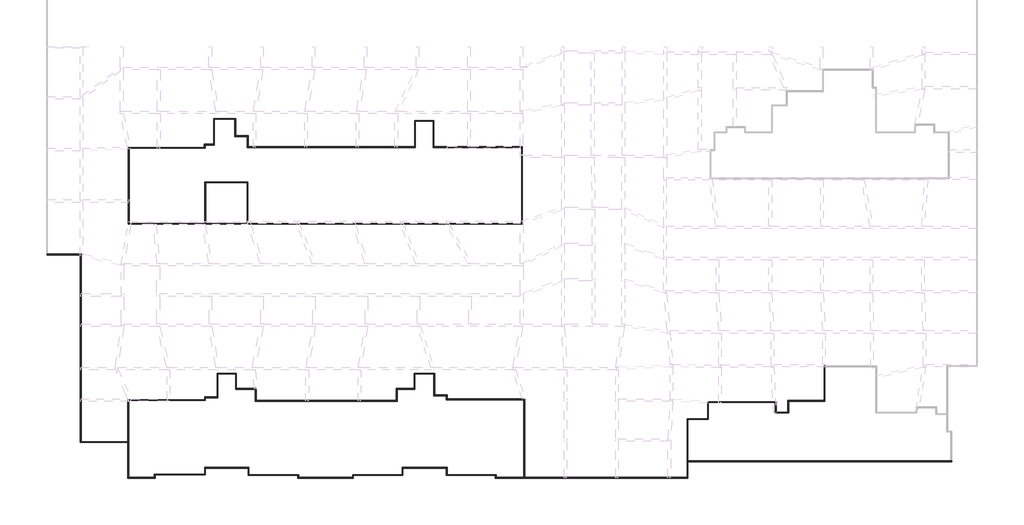
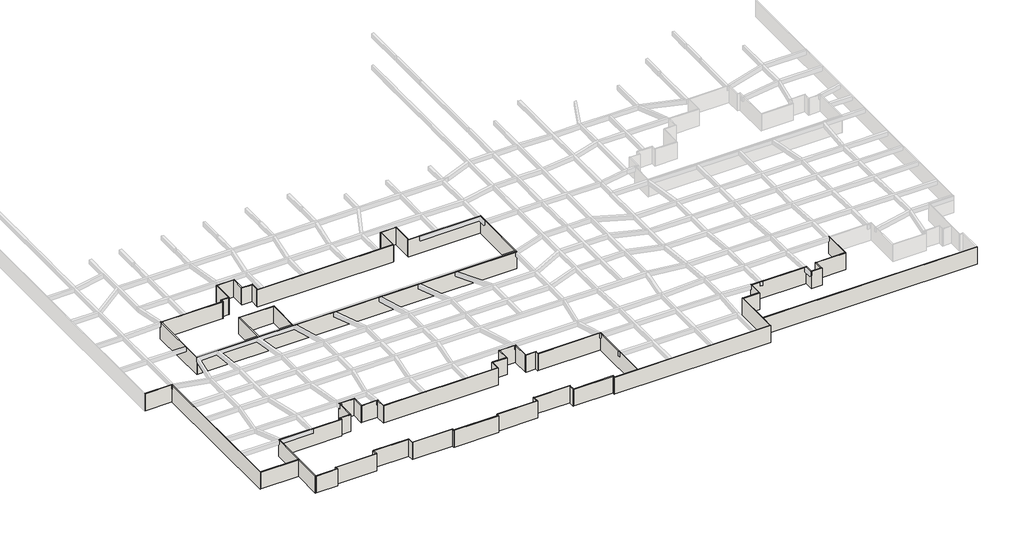
# One storey, part 1 of 45: 68 walls.
"""IFC4 building model written with IfcOpenShell, lengths in millimetres."""

from ifc_helpers import new_model, si_unit, origin, origin_with_axes, place, context, project, spatial, polyline, outline, extrude, faceted_brep, element, save

model = new_model("IFC4")

# Units and contexts
model_context = context("Model", 3, world=origin())
ifc_project = project(units=[si_unit("LENGTHUNIT", "METRE", prefix="MILLI")], contexts=[model_context])

# Site, building, storey
site = spatial("IfcSite", under=ifc_project)
building = spatial("IfcBuilding", under=site)
storey = spatial("IfcBuildingStorey", under=building, Name="户型图", Elevation=0.0)

# Walls
placement = place(None, origin())
element("IfcWall", 1, ObjectType="所有墙体", at=placement, inside=storey, context=model_context, shape_type="Brep", body=[
    faceted_brep([(-145580.5216564, -158288.0123265, 0.0), (-140600.5216564, -158288.0123265, 0.0), (-140480.5216564, -158288.0123265, 0.0), (-140480.5216564, -158288.0123265, 3300.0), (-140600.5216564, -158288.0123265, 3300.0), (-145580.5216564, -158288.0123265, 3300.0), (-145580.5216564, -158168.0123265, 0.0), (-145580.5216564, -158168.0123265, 3300.0), (-140480.5216564, -158168.0123265, 3300.0), (-140480.5216564, -158168.0123265, 0.0)], [[[0, 1, 2, 3, 4, 5]], [[6, 7, 8, 9]], [[2, 1, 0, 6, 9]], [[5, 4, 3, 8, 7]], [[0, 5, 7, 6]], [[3, 2, 9, 8]]]),
])
element("IfcWall", 2, ObjectType="所有墙体", at=placement, inside=storey, context=model_context, shape_type="Brep", body=[
    faceted_brep([(-140600.5216564, -158288.0123265, 0.0), (-140600.5216564, -186688.0123265, 0.0), (-140600.5216564, -186688.0123265, 3300.0), (-140600.5216564, -158288.0123265, 3300.0), (-140480.5216564, -158288.0123265, 0.0), (-140480.5216564, -158288.0123265, 3300.0), (-140480.5216564, -186568.0123265, 3300.0), (-140480.5216564, -186688.0123265, 3300.0), (-140480.5216564, -186688.0123265, 0.0), (-140480.5216564, -186568.0123265, 0.0)], [[[0, 1, 2, 3]], [[4, 5, 6, 7, 8, 9]], [[1, 0, 4, 9, 8]], [[3, 2, 7, 6, 5]], [[0, 3, 5, 4]], [[2, 1, 8, 7]]]),
])
element("IfcWall", 3, ObjectType="所有墙体", at=placement, inside=storey, context=model_context, shape_type="SweptSolid", body=[
    extrude(outline(polyline([(-133400.5216564, -186688.0123265), (-140480.5216564, -186688.0123265), (-140480.5216564, -186568.0123265), (-133400.5216564, -186568.0123265), (-133400.5216564, -186688.0123265)])), origin_with_axes(), (0.0, 0.0, 1.0), 3300.0),
])
element("IfcWall", 4, ObjectType="所有墙体", at=placement, inside=storey, context=model_context, shape_type="Brep", body=[
    faceted_brep([(-133400.5216564, -180210.4346237, 0.0), (-133400.5216564, -186568.0123265, 0.0), (-133400.5216564, -186688.0123265, 0.0), (-133400.5216564, -192088.0123265, 0.0), (-133400.5216564, -192088.0123265, 3300.0), (-133400.5216564, -186688.0123265, 3300.0), (-133400.5216564, -186568.0123265, 3300.0), (-133400.5216564, -180210.4346237, 3300.0), (-133280.5216564, -180210.4346237, 0.0), (-133280.5216564, -180210.4346237, 3300.0), (-133280.5216564, -180330.4346237, 3300.0), (-133280.5216564, -191968.0123265, 3300.0), (-133280.5216564, -192088.0123265, 3300.0), (-133280.5216564, -192088.0123265, 0.0), (-133280.5216564, -191968.0123265, 0.0), (-133280.5216564, -180330.4346237, 0.0)], [[[0, 1, 2, 3, 4, 5, 6, 7]], [[8, 9, 10, 11, 12, 13, 14, 15]], [[3, 2, 1, 0, 8, 15, 14, 13]], [[7, 6, 5, 4, 12, 11, 10, 9]], [[4, 3, 13, 12]], [[0, 7, 9, 8]]]),
])
element("IfcWall", 5, ObjectType="所有墙体", at=placement, inside=storey, context=model_context, shape_type="Brep", body=[
    faceted_brep([(-133280.5216564, -192088.0123265, 0.0), (-129280.5216564, -192088.0123265, 0.0), (-129280.5216564, -192088.0123265, 3300.0), (-133280.5216564, -192088.0123265, 3300.0), (-133280.5216564, -191968.0123265, 0.0), (-133280.5216564, -191968.0123265, 3300.0), (-129400.5216564, -191968.0123265, 3300.0), (-129280.5216564, -191968.0123265, 3300.0), (-129280.5216564, -191968.0123265, 0.0), (-129400.5216564, -191968.0123265, 0.0)], [[[0, 1, 2, 3]], [[4, 5, 6, 7, 8, 9]], [[1, 0, 4, 9, 8]], [[3, 2, 7, 6, 5]], [[0, 3, 5, 4]], [[2, 1, 8, 7]]]),
])
element("IfcWall", 6, ObjectType="所有墙体", at=placement, inside=storey, context=model_context, shape_type="Brep", body=[
    faceted_brep([(-129280.5216564, -191968.0123265, 0.0), (-129280.5216564, -191588.0123265, 0.0), (-129280.5216564, -191468.0123265, 0.0), (-129280.5216564, -191468.0123265, 3300.0), (-129280.5216564, -191588.0123265, 3300.0), (-129280.5216564, -191968.0123265, 3300.0), (-129400.5216564, -191968.0123265, 0.0), (-129400.5216564, -191968.0123265, 3300.0), (-129400.5216564, -191468.0123265, 3300.0), (-129400.5216564, -191468.0123265, 0.0)], [[[0, 1, 2, 3, 4, 5]], [[6, 7, 8, 9]], [[2, 1, 0, 6, 9]], [[5, 4, 3, 8, 7]], [[0, 5, 7, 6]], [[3, 2, 9, 8]]]),
])
element("IfcWall", 7, ObjectType="所有墙体", at=placement, inside=storey, context=model_context, shape_type="Brep", body=[
    faceted_brep([(-129280.5216564, -191588.0123265, 0.0), (-121680.5216564, -191588.0123265, 0.0), (-121680.5216564, -191588.0123265, 3300.0), (-129280.5216564, -191588.0123265, 3300.0), (-129280.5216564, -191468.0123265, 0.0), (-129280.5216564, -191468.0123265, 3300.0), (-121800.5216564, -191468.0123265, 3300.0), (-121680.5216564, -191468.0123265, 3300.0), (-121680.5216564, -191468.0123265, 0.0), (-121800.5216564, -191468.0123265, 0.0)], [[[0, 1, 2, 3]], [[4, 5, 6, 7, 8, 9]], [[1, 0, 4, 9, 8]], [[3, 2, 7, 6, 5]], [[0, 3, 5, 4]], [[2, 1, 8, 7]]]),
])
element("IfcWall", 8, ObjectType="所有墙体", at=placement, inside=storey, context=model_context, shape_type="Brep", body=[
    faceted_brep([(-121680.5216564, -191468.0123265, 0.0), (-121680.5216564, -190588.0123265, 0.0), (-121680.5216564, -190468.0123265, 0.0), (-121680.5216564, -190468.0123265, 3300.0), (-121680.5216564, -190588.0123265, 3300.0), (-121680.5216564, -191468.0123265, 3300.0), (-121800.5216564, -191468.0123265, 0.0), (-121800.5216564, -191468.0123265, 3300.0), (-121800.5216564, -190468.0123265, 3300.0), (-121800.5216564, -190468.0123265, 0.0)], [[[0, 1, 2, 3, 4, 5]], [[6, 7, 8, 9]], [[2, 1, 0, 6, 9]], [[5, 4, 3, 8, 7]], [[0, 5, 7, 6]], [[3, 2, 9, 8]]]),
])
element("IfcWall", 9, ObjectType="所有墙体", at=placement, inside=storey, context=model_context, shape_type="Brep", body=[
    faceted_brep([(-121680.5216564, -190588.0123265, 0.0), (-115200.5216564, -190588.0123265, 0.0), (-115080.5216564, -190588.0123265, 0.0), (-115080.5216564, -190588.0123265, 3300.0), (-115200.5216564, -190588.0123265, 3300.0), (-121680.5216564, -190588.0123265, 3300.0), (-121680.5216564, -190468.0123265, 0.0), (-121680.5216564, -190468.0123265, 3300.0), (-115080.5216564, -190468.0123265, 3300.0), (-115080.5216564, -190468.0123265, 0.0)], [[[0, 1, 2, 3, 4, 5]], [[6, 7, 8, 9]], [[2, 1, 0, 6, 9]], [[5, 4, 3, 8, 7]], [[0, 5, 7, 6]], [[3, 2, 9, 8]]]),
])
element("IfcWall", 10, ObjectType="所有墙体", at=placement, inside=storey, context=model_context, shape_type="Brep", body=[
    faceted_brep([(-115200.5216564, -190588.0123265, 0.0), (-115200.5216564, -191688.0123265, 0.0), (-115200.5216564, -191688.0123265, 3300.0), (-115200.5216564, -190588.0123265, 3300.0), (-115080.5216564, -190588.0123265, 0.0), (-115080.5216564, -190588.0123265, 3300.0), (-115080.5216564, -191568.0123265, 3300.0), (-115080.5216564, -191688.0123265, 3300.0), (-115080.5216564, -191688.0123265, 0.0), (-115080.5216564, -191568.0123265, 0.0)], [[[0, 1, 2, 3]], [[4, 5, 6, 7, 8, 9]], [[1, 0, 4, 9, 8]], [[3, 2, 7, 6, 5]], [[0, 3, 5, 4]], [[2, 1, 8, 7]]]),
])
element("IfcWall", 11, ObjectType="所有墙体", at=placement, inside=storey, context=model_context, shape_type="Brep", body=[
    faceted_brep([(-115080.5216564, -191688.0123265, 0.0), (-107700.5216564, -191688.0123265, 0.0), (-107580.5216564, -191688.0123265, 0.0), (-107580.5216564, -191688.0123265, 3300.0), (-107700.5216564, -191688.0123265, 3300.0), (-115080.5216564, -191688.0123265, 3300.0), (-115080.5216564, -191568.0123265, 0.0), (-115080.5216564, -191568.0123265, 3300.0), (-107580.5216564, -191568.0123265, 3300.0), (-107580.5216564, -191568.0123265, 0.0)], [[[0, 1, 2, 3, 4, 5]], [[6, 7, 8, 9]], [[2, 1, 0, 6, 9]], [[5, 4, 3, 8, 7]], [[0, 5, 7, 6]], [[3, 2, 9, 8]]]),
])
element("IfcWall", 12, ObjectType="所有墙体", at=placement, inside=storey, context=model_context, shape_type="Brep", body=[
    faceted_brep([(-107700.5216564, -191688.0123265, 0.0), (-107700.5216564, -192088.0123265, 0.0), (-107700.5216564, -192088.0123265, 3300.0), (-107700.5216564, -191688.0123265, 3300.0), (-107580.5216564, -191688.0123265, 0.0), (-107580.5216564, -191688.0123265, 3300.0), (-107580.5216564, -191968.0123265, 3300.0), (-107580.5216564, -192088.0123265, 3300.0), (-107580.5216564, -192088.0123265, 0.0), (-107580.5216564, -191968.0123265, 0.0)], [[[0, 1, 2, 3]], [[4, 5, 6, 7, 8, 9]], [[1, 0, 4, 9, 8]], [[3, 2, 7, 6, 5]], [[0, 3, 5, 4]], [[2, 1, 8, 7]]]),
])
element("IfcWall", 13, ObjectType="所有墙体", at=placement, inside=storey, context=model_context, shape_type="Brep", body=[
    faceted_brep([(-107580.5216564, -192088.0123265, 0.0), (-99280.5216564, -192088.0123265, 0.0), (-99280.5216564, -192088.0123265, 3300.0), (-107580.5216564, -192088.0123265, 3300.0), (-107580.5216564, -191968.0123265, 0.0), (-107580.5216564, -191968.0123265, 3300.0), (-99400.5216564, -191968.0123265, 3300.0), (-99280.5216564, -191968.0123265, 3300.0), (-99280.5216564, -191968.0123265, 0.0), (-99400.5216564, -191968.0123265, 0.0)], [[[0, 1, 2, 3]], [[4, 5, 6, 7, 8, 9]], [[1, 0, 4, 9, 8]], [[3, 2, 7, 6, 5]], [[0, 3, 5, 4]], [[2, 1, 8, 7]]]),
])
element("IfcWall", 14, ObjectType="所有墙体", at=placement, inside=storey, context=model_context, shape_type="Brep", body=[
    faceted_brep([(-99280.5216564, -191968.0123265, 0.0), (-99280.5216564, -191688.0123265, 0.0), (-99280.5216564, -191568.0123265, 0.0), (-99280.5216564, -191568.0123265, 3300.0), (-99280.5216564, -191688.0123265, 3300.0), (-99280.5216564, -191968.0123265, 3300.0), (-99400.5216564, -191968.0123265, 0.0), (-99400.5216564, -191968.0123265, 3300.0), (-99400.5216564, -191568.0123265, 3300.0), (-99400.5216564, -191568.0123265, 0.0)], [[[0, 1, 2, 3, 4, 5]], [[6, 7, 8, 9]], [[2, 1, 0, 6, 9]], [[5, 4, 3, 8, 7]], [[0, 5, 7, 6]], [[3, 2, 9, 8]]]),
])
element("IfcWall", 15, ObjectType="所有墙体", at=placement, inside=storey, context=model_context, shape_type="Brep", body=[
    faceted_brep([(-99280.5216564, -191688.0123265, 0.0), (-91780.5216564, -191688.0123265, 0.0), (-91780.5216564, -191688.0123265, 3300.0), (-99280.5216564, -191688.0123265, 3300.0), (-99280.5216564, -191568.0123265, 0.0), (-99280.5216564, -191568.0123265, 3300.0), (-91900.5216564, -191568.0123265, 3300.0), (-91780.5216564, -191568.0123265, 3300.0), (-91780.5216564, -191568.0123265, 0.0), (-91900.5216564, -191568.0123265, 0.0)], [[[0, 1, 2, 3]], [[4, 5, 6, 7, 8, 9]], [[1, 0, 4, 9, 8]], [[3, 2, 7, 6, 5]], [[0, 3, 5, 4]], [[2, 1, 8, 7]]]),
])
element("IfcWall", 16, ObjectType="所有墙体", at=placement, inside=storey, context=model_context, shape_type="Brep", body=[
    faceted_brep([(-91780.5216564, -191568.0123265, 0.0), (-91780.5216564, -190588.0123265, 0.0), (-91780.5216564, -190468.0123265, 0.0), (-91780.5216564, -190468.0123265, 3300.0), (-91780.5216564, -190588.0123265, 3300.0), (-91780.5216564, -191568.0123265, 3300.0), (-91900.5216564, -191568.0123265, 0.0), (-91900.5216564, -191568.0123265, 3300.0), (-91900.5216564, -190468.0123265, 3300.0), (-91900.5216564, -190468.0123265, 0.0)], [[[0, 1, 2, 3, 4, 5]], [[6, 7, 8, 9]], [[2, 1, 0, 6, 9]], [[5, 4, 3, 8, 7]], [[0, 5, 7, 6]], [[3, 2, 9, 8]]]),
])
element("IfcWall", 17, ObjectType="所有墙体", at=placement, inside=storey, context=model_context, shape_type="Brep", body=[
    faceted_brep([(-91780.5216564, -190588.0123265, 0.0), (-85200.5216564, -190588.0123265, 0.0), (-85080.5216564, -190588.0123265, 0.0), (-85080.5216564, -190588.0123265, 3300.0), (-85200.5216564, -190588.0123265, 3300.0), (-91780.5216564, -190588.0123265, 3300.0), (-91780.5216564, -190468.0123265, 0.0), (-91780.5216564, -190468.0123265, 3300.0), (-85080.5216564, -190468.0123265, 3300.0), (-85080.5216564, -190468.0123265, 0.0)], [[[0, 1, 2, 3, 4, 5]], [[6, 7, 8, 9]], [[2, 1, 0, 6, 9]], [[5, 4, 3, 8, 7]], [[0, 5, 7, 6]], [[3, 2, 9, 8]]]),
])
element("IfcWall", 18, ObjectType="所有墙体", at=placement, inside=storey, context=model_context, shape_type="Brep", body=[
    faceted_brep([(-85200.5216564, -190588.0123265, 0.0), (-85200.5216564, -191688.0123265, 0.0), (-85200.5216564, -191688.0123265, 3300.0), (-85200.5216564, -190588.0123265, 3300.0), (-85080.5216564, -190588.0123265, 0.0), (-85080.5216564, -190588.0123265, 3300.0), (-85080.5216564, -191568.0123265, 3300.0), (-85080.5216564, -191688.0123265, 3300.0), (-85080.5216564, -191688.0123265, 0.0), (-85080.5216564, -191568.0123265, 0.0)], [[[0, 1, 2, 3]], [[4, 5, 6, 7, 8, 9]], [[1, 0, 4, 9, 8]], [[3, 2, 7, 6, 5]], [[0, 3, 5, 4]], [[2, 1, 8, 7]]]),
])
element("IfcWall", 19, ObjectType="所有墙体", at=placement, inside=storey, context=model_context, shape_type="Brep", body=[
    faceted_brep([(-85080.5216564, -191688.0123265, 0.0), (-77800.5216564, -191688.0123265, 0.0), (-77680.5216564, -191688.0123265, 0.0), (-77680.5216564, -191688.0123265, 3300.0), (-77800.5216564, -191688.0123265, 3300.0), (-85080.5216564, -191688.0123265, 3300.0), (-85080.5216564, -191568.0123265, 0.0), (-85080.5216564, -191568.0123265, 3300.0), (-77680.5216564, -191568.0123265, 3300.0), (-77680.5216564, -191568.0123265, 0.0)], [[[0, 1, 2, 3, 4, 5]], [[6, 7, 8, 9]], [[2, 1, 0, 6, 9]], [[5, 4, 3, 8, 7]], [[0, 5, 7, 6]], [[3, 2, 9, 8]]]),
])
element("IfcWall", 20, ObjectType="所有墙体", at=placement, inside=storey, context=model_context, shape_type="Brep", body=[
    faceted_brep([(-77800.5216564, -191688.0123265, 0.0), (-77800.5216564, -192088.0123265, 0.0), (-77800.5216564, -192088.0123265, 3300.0), (-77800.5216564, -191688.0123265, 3300.0), (-77680.5216564, -191688.0123265, 0.0), (-77680.5216564, -191688.0123265, 3300.0), (-77680.5216564, -191968.0123265, 3300.0), (-77680.5216564, -192088.0123265, 3300.0), (-77680.5216564, -192088.0123265, 0.0), (-77680.5216564, -191968.0123265, 0.0)], [[[0, 1, 2, 3]], [[4, 5, 6, 7, 8, 9]], [[1, 0, 4, 9, 8]], [[3, 2, 7, 6, 5]], [[0, 3, 5, 4]], [[2, 1, 8, 7]]]),
])
element("IfcWall", 21, ObjectType="所有墙体", at=placement, inside=storey, context=model_context, shape_type="Brep", body=[
    faceted_brep([(-77680.5216564, -192088.0123265, 0.0), (-48680.5216564, -192088.0123265, 0.0), (-48680.5216564, -192088.0123265, 3300.0), (-77680.5216564, -192088.0123265, 3300.0), (-77680.5216564, -191968.0123265, 0.0), (-77680.5216564, -191968.0123265, 3300.0), (-73500.5216564, -191968.0123265, 3300.0), (-73380.5216564, -191968.0123265, 3300.0), (-48800.5216564, -191968.0123265, 3300.0), (-48680.5216564, -191968.0123265, 3300.0), (-48680.5216564, -191968.0123265, 0.0), (-48800.5216564, -191968.0123265, 0.0), (-73380.5216564, -191968.0123265, 0.0), (-73500.5216564, -191968.0123265, 0.0)], [[[0, 1, 2, 3]], [[4, 5, 6, 7, 8, 9, 10, 11, 12, 13]], [[1, 0, 4, 13, 12, 11, 10]], [[3, 2, 9, 8, 7, 6, 5]], [[0, 3, 5, 4]], [[2, 1, 10, 9]]]),
])
element("IfcWall", 22, ObjectType="所有墙体", at=placement, inside=storey, context=model_context, shape_type="Brep", body=[
    faceted_brep([(-48680.5216564, -191968.0123265, 0.0), (-48680.5216564, -189588.0123265, 0.0), (-48680.5216564, -189468.0123265, 0.0), (-48680.5216564, -183188.0123265, 0.0), (-48680.5216564, -183068.0123265, 0.0), (-48680.5216564, -183068.0123265, 3300.0), (-48680.5216564, -183188.0123265, 3300.0), (-48680.5216564, -189468.0123265, 3300.0), (-48680.5216564, -189588.0123265, 3300.0), (-48680.5216564, -191968.0123265, 3300.0), (-48800.5216564, -191968.0123265, 0.0), (-48800.5216564, -191968.0123265, 3300.0), (-48800.5216564, -183068.0123265, 3300.0), (-48800.5216564, -183068.0123265, 0.0)], [[[0, 1, 2, 3, 4, 5, 6, 7, 8, 9]], [[10, 11, 12, 13]], [[4, 3, 2, 1, 0, 10, 13]], [[9, 8, 7, 6, 5, 12, 11]], [[0, 9, 11, 10]], [[5, 4, 13, 12]]]),
])
element("IfcWall", 23, ObjectType="所有墙体", at=placement, inside=storey, context=model_context, shape_type="Brep", body=[
    faceted_brep([(-48680.5216564, -189588.0123265, 0.0), (-8780.5216564, -189588.0123265, 0.0), (-8780.5216564, -189588.0123265, 3300.0), (-48680.5216564, -189588.0123265, 3300.0), (-48680.5216564, -189468.0123265, 0.0), (-48680.5216564, -189468.0123265, 3300.0), (-8900.5216564, -189468.0123265, 3300.0), (-8780.5216564, -189468.0123265, 3300.0), (-8780.5216564, -189468.0123265, 0.0), (-8900.5216564, -189468.0123265, 0.0)], [[[0, 1, 2, 3]], [[4, 5, 6, 7, 8, 9]], [[1, 0, 4, 9, 8]], [[3, 2, 7, 6, 5]], [[0, 3, 5, 4]], [[2, 1, 8, 7]]]),
])
element("IfcWall", 24, ObjectType="所有墙体", at=placement, inside=storey, context=model_context, shape_type="Brep", body=[
    faceted_brep([(-133280.5216564, -180330.4346237, 0.0), (-121680.5216564, -180330.4346237, 0.0), (-121680.5216564, -180330.4346237, 3300.0), (-133280.5216564, -180330.4346237, 3300.0), (-133280.5216564, -180210.4346237, 0.0), (-133280.5216564, -180210.4346237, 3300.0), (-121800.5216564, -180210.4346237, 3300.0), (-121680.5216564, -180210.4346237, 3300.0), (-121680.5216564, -180210.4346237, 0.0), (-121800.5216564, -180210.4346237, 0.0)], [[[0, 1, 2, 3]], [[4, 5, 6, 7, 8, 9]], [[1, 0, 4, 9, 8]], [[3, 2, 7, 6, 5]], [[0, 3, 5, 4]], [[2, 1, 8, 7]]]),
])
element("IfcWall", 25, ObjectType="所有墙体", at=placement, inside=storey, context=model_context, shape_type="Brep", body=[
    faceted_brep([(-121680.5216564, -180210.4346237, 0.0), (-121680.5216564, -179930.4346237, 0.0), (-121680.5216564, -179810.4346237, 0.0), (-121680.5216564, -179810.4346237, 3300.0), (-121680.5216564, -179930.4346237, 3300.0), (-121680.5216564, -180210.4346237, 3300.0), (-121800.5216564, -180210.4346237, 0.0), (-121800.5216564, -180210.4346237, 3300.0), (-121800.5216564, -179810.4346237, 3300.0), (-121800.5216564, -179810.4346237, 0.0)], [[[0, 1, 2, 3, 4, 5]], [[6, 7, 8, 9]], [[2, 1, 0, 6, 9]], [[5, 4, 3, 8, 7]], [[0, 5, 7, 6]], [[3, 2, 9, 8]]]),
])
element("IfcWall", 26, ObjectType="所有墙体", at=placement, inside=storey, context=model_context, shape_type="Brep", body=[
    faceted_brep([(-121680.5216564, -179930.4346237, 0.0), (-119780.5216564, -179930.4346237, 0.0), (-119780.5216564, -179930.4346237, 3300.0), (-121680.5216564, -179930.4346237, 3300.0), (-121680.5216564, -179810.4346237, 0.0), (-121680.5216564, -179810.4346237, 3300.0), (-119900.5216564, -179810.4346237, 3300.0), (-119780.5216564, -179810.4346237, 3300.0), (-119780.5216564, -179810.4346237, 0.0), (-119900.5216564, -179810.4346237, 0.0)], [[[0, 1, 2, 3]], [[4, 5, 6, 7, 8, 9]], [[1, 0, 4, 9, 8]], [[3, 2, 7, 6, 5]], [[0, 3, 5, 4]], [[2, 1, 8, 7]]]),
])
element("IfcWall", 27, ObjectType="所有墙体", at=placement, inside=storey, context=model_context, shape_type="Brep", body=[
    faceted_brep([(-119780.5216564, -179810.4346237, 0.0), (-119780.5216564, -176330.4346237, 0.0), (-119780.5216564, -176210.4346237, 0.0), (-119780.5216564, -176210.4346237, 3300.0), (-119780.5216564, -176330.4346237, 3300.0), (-119780.5216564, -179810.4346237, 3300.0), (-119900.5216564, -179810.4346237, 0.0), (-119900.5216564, -179810.4346237, 3300.0), (-119900.5216564, -176210.4346237, 3300.0), (-119900.5216564, -176210.4346237, 0.0)], [[[0, 1, 2, 3, 4, 5]], [[6, 7, 8, 9]], [[2, 1, 0, 6, 9]], [[5, 4, 3, 8, 7]], [[0, 5, 7, 6]], [[3, 2, 9, 8]]]),
])
element("IfcWall", 28, ObjectType="所有墙体", at=placement, inside=storey, context=model_context, shape_type="Brep", body=[
    faceted_brep([(-119780.5216564, -176330.4346237, 0.0), (-117100.5216564, -176330.4346237, 0.0), (-116980.5216564, -176330.4346237, 0.0), (-116980.5216564, -176330.4346237, 3300.0), (-117100.5216564, -176330.4346237, 3300.0), (-119780.5216564, -176330.4346237, 3300.0), (-119780.5216564, -176210.4346237, 0.0), (-119780.5216564, -176210.4346237, 3300.0), (-116980.5216564, -176210.4346237, 3300.0), (-116980.5216564, -176210.4346237, 0.0)], [[[0, 1, 2, 3, 4, 5]], [[6, 7, 8, 9]], [[2, 1, 0, 6, 9]], [[5, 4, 3, 8, 7]], [[0, 5, 7, 6]], [[3, 2, 9, 8]]]),
])
element("IfcWall", 29, ObjectType="所有墙体", at=placement, inside=storey, context=model_context, shape_type="Brep", body=[
    faceted_brep([(-117100.5216564, -176330.4346237, 0.0), (-117100.5216564, -178630.4346237, 0.0), (-117100.5216564, -178630.4346237, 3300.0), (-117100.5216564, -176330.4346237, 3300.0), (-116980.5216564, -176330.4346237, 0.0), (-116980.5216564, -176330.4346237, 3300.0), (-116980.5216564, -178510.4346237, 3300.0), (-116980.5216564, -178630.4346237, 3300.0), (-116980.5216564, -178630.4346237, 0.0), (-116980.5216564, -178510.4346237, 0.0)], [[[0, 1, 2, 3]], [[4, 5, 6, 7, 8, 9]], [[1, 0, 4, 9, 8]], [[3, 2, 7, 6, 5]], [[0, 3, 5, 4]], [[2, 1, 8, 7]]]),
])
element("IfcWall", 30, ObjectType="所有墙体", at=placement, inside=storey, context=model_context, shape_type="Brep", body=[
    faceted_brep([(-116980.5216564, -178630.4346237, 0.0), (-114100.5216564, -178630.4346237, 0.0), (-113980.5216564, -178630.4346237, 0.0), (-113980.5216564, -178630.4346237, 3300.0), (-114100.5216564, -178630.4346237, 3300.0), (-116980.5216564, -178630.4346237, 3300.0), (-116980.5216564, -178510.4346237, 0.0), (-116980.5216564, -178510.4346237, 3300.0), (-113980.5216564, -178510.4346237, 3300.0), (-113980.5216564, -178510.4346237, 0.0)], [[[0, 1, 2, 3, 4, 5]], [[6, 7, 8, 9]], [[2, 1, 0, 6, 9]], [[5, 4, 3, 8, 7]], [[0, 5, 7, 6]], [[3, 2, 9, 8]]]),
])
element("IfcWall", 31, ObjectType="所有墙体", at=placement, inside=storey, context=model_context, shape_type="Brep", body=[
    faceted_brep([(-114100.5216564, -178630.4346237, 0.0), (-114100.5216564, -180430.4346237, 0.0), (-114100.5216564, -180430.4346237, 3300.0), (-114100.5216564, -178630.4346237, 3300.0), (-113980.5216564, -178630.4346237, 0.0), (-113980.5216564, -178630.4346237, 3300.0), (-113980.5216564, -180310.4346237, 3300.0), (-113980.5216564, -180430.4346237, 3300.0), (-113980.5216564, -180430.4346237, 0.0), (-113980.5216564, -180310.4346237, 0.0)], [[[0, 1, 2, 3]], [[4, 5, 6, 7, 8, 9]], [[1, 0, 4, 9, 8]], [[3, 2, 7, 6, 5]], [[0, 3, 5, 4]], [[2, 1, 8, 7]]]),
])
element("IfcWall", 32, ObjectType="所有墙体", at=placement, inside=storey, context=model_context, shape_type="Brep", body=[
    faceted_brep([(-113980.5216564, -180430.4346237, 0.0), (-92680.5216564, -180430.4346237, 0.0), (-92680.5216564, -180430.4346237, 3300.0), (-113980.5216564, -180430.4346237, 3300.0), (-113980.5216564, -180310.4346237, 0.0), (-113980.5216564, -180310.4346237, 3300.0), (-92800.5216564, -180310.4346237, 3300.0), (-92680.5216564, -180310.4346237, 3300.0), (-92680.5216564, -180310.4346237, 0.0), (-92800.5216564, -180310.4346237, 0.0)], [[[0, 1, 2, 3]], [[4, 5, 6, 7, 8, 9]], [[1, 0, 4, 9, 8]], [[3, 2, 7, 6, 5]], [[0, 3, 5, 4]], [[2, 1, 8, 7]]]),
])
element("IfcWall", 33, ObjectType="所有墙体", at=placement, inside=storey, context=model_context, shape_type="Brep", body=[
    faceted_brep([(-92680.5216564, -180310.4346237, 0.0), (-92680.5216564, -178630.4346237, 0.0), (-92680.5216564, -178510.4346237, 0.0), (-92680.5216564, -178510.4346237, 3300.0), (-92680.5216564, -178630.4346237, 3300.0), (-92680.5216564, -180310.4346237, 3300.0), (-92800.5216564, -180310.4346237, 0.0), (-92800.5216564, -180310.4346237, 3300.0), (-92800.5216564, -178510.4346237, 3300.0), (-92800.5216564, -178510.4346237, 0.0)], [[[0, 1, 2, 3, 4, 5]], [[6, 7, 8, 9]], [[2, 1, 0, 6, 9]], [[5, 4, 3, 8, 7]], [[0, 5, 7, 6]], [[3, 2, 9, 8]]]),
])
element("IfcWall", 34, ObjectType="所有墙体", at=placement, inside=storey, context=model_context, shape_type="Brep", body=[
    faceted_brep([(-92680.5216564, -178630.4346237, 0.0), (-89980.5216564, -178630.4346237, 0.0), (-89980.5216564, -178630.4346237, 3300.0), (-92680.5216564, -178630.4346237, 3300.0), (-92680.5216564, -178510.4346237, 0.0), (-92680.5216564, -178510.4346237, 3300.0), (-90100.5216564, -178510.4346237, 3300.0), (-89980.5216564, -178510.4346237, 3300.0), (-89980.5216564, -178510.4346237, 0.0), (-90100.5216564, -178510.4346237, 0.0)], [[[0, 1, 2, 3]], [[4, 5, 6, 7, 8, 9]], [[1, 0, 4, 9, 8]], [[3, 2, 7, 6, 5]], [[0, 3, 5, 4]], [[2, 1, 8, 7]]]),
])
element("IfcWall", 35, ObjectType="所有墙体", at=placement, inside=storey, context=model_context, shape_type="Brep", body=[
    faceted_brep([(-89980.5216564, -178510.4346237, 0.0), (-89980.5216564, -176330.4346237, 0.0), (-89980.5216564, -176210.4346237, 0.0), (-89980.5216564, -176210.4346237, 3300.0), (-89980.5216564, -176330.4346237, 3300.0), (-89980.5216564, -178510.4346237, 3300.0), (-90100.5216564, -178510.4346237, 0.0), (-90100.5216564, -178510.4346237, 3300.0), (-90100.5216564, -176210.4346237, 3300.0), (-90100.5216564, -176210.4346237, 0.0)], [[[0, 1, 2, 3, 4, 5]], [[6, 7, 8, 9]], [[2, 1, 0, 6, 9]], [[5, 4, 3, 8, 7]], [[0, 5, 7, 6]], [[3, 2, 9, 8]]]),
])
element("IfcWall", 36, ObjectType="所有墙体", at=placement, inside=storey, context=model_context, shape_type="Brep", body=[
    faceted_brep([(-89980.5216564, -176330.4346237, 0.0), (-87098.9727528, -176330.4346237, 0.0), (-86978.9727528, -176330.4346237, 0.0), (-86978.9727528, -176330.4346237, 3300.0), (-87098.9727528, -176330.4346237, 3300.0), (-89980.5216564, -176330.4346237, 3300.0), (-89980.5216564, -176210.4346237, 0.0), (-89980.5216564, -176210.4346237, 3300.0), (-86978.9727528, -176210.4346237, 3300.0), (-86978.9727528, -176210.4346237, 0.0)], [[[0, 1, 2, 3, 4, 5]], [[6, 7, 8, 9]], [[2, 1, 0, 6, 9]], [[5, 4, 3, 8, 7]], [[0, 5, 7, 6]], [[3, 2, 9, 8]]]),
])
element("IfcWall", 37, ObjectType="所有墙体", at=placement, inside=storey, context=model_context, shape_type="SweptSolid", body=[
    extrude(outline(polyline([(-87098.9727528, -179475.6864738), (-87098.9727528, -176330.4346237), (-86978.9727528, -176330.4346237), (-86978.9727528, -179475.6864738), (-87098.9727528, -179475.6864738)])), origin_with_axes(), (0.0, 0.0, 1.0), 3300.0),
])
element("IfcWall", 38, ObjectType="所有墙体", at=placement, inside=storey, context=model_context, shape_type="Brep", body=[
    faceted_brep([(-87098.9727528, -179595.6864738, 0.0), (-85200.5216564, -179595.6864738, 0.0), (-85080.5216564, -179595.6864738, 0.0), (-85080.5216564, -179595.6864738, 3300.0), (-85200.5216564, -179595.6864738, 3300.0), (-87098.9727528, -179595.6864738, 3300.0), (-87098.9727528, -179475.6864738, 0.0), (-87098.9727528, -179475.6864738, 3300.0), (-86978.9727528, -179475.6864738, 3300.0), (-85080.5216564, -179475.6864738, 3300.0), (-85080.5216564, -179475.6864738, 0.0), (-86978.9727528, -179475.6864738, 0.0)], [[[0, 1, 2, 3, 4, 5]], [[6, 7, 8, 9, 10, 11]], [[2, 1, 0, 6, 11, 10]], [[5, 4, 3, 9, 8, 7]], [[3, 2, 10, 9]], [[0, 5, 7, 6]]]),
])
element("IfcWall", 39, ObjectType="所有墙体", at=placement, inside=storey, context=model_context, shape_type="Brep", body=[
    faceted_brep([(-85200.5216564, -179595.6864738, 0.0), (-85200.5216564, -180195.6864738, 0.0), (-85200.5216564, -180195.6864738, 3300.0), (-85200.5216564, -179595.6864738, 3300.0), (-85080.5216564, -179595.6864738, 0.0), (-85080.5216564, -179595.6864738, 3300.0), (-85080.5216564, -180075.6864738, 3300.0), (-85080.5216564, -180195.6864738, 3300.0), (-85080.5216564, -180195.6864738, 0.0), (-85080.5216564, -180075.6864738, 0.0)], [[[0, 1, 2, 3]], [[4, 5, 6, 7, 8, 9]], [[1, 0, 4, 9, 8]], [[3, 2, 7, 6, 5]], [[0, 3, 5, 4]], [[2, 1, 8, 7]]]),
])
element("IfcWall", 40, ObjectType="所有墙体", at=placement, inside=storey, context=model_context, shape_type="Brep", body=[
    faceted_brep([(-85080.5216564, -180195.6864738, 0.0), (-73500.5216564, -180195.6864738, 0.0), (-73380.5216564, -180195.6864738, 0.0), (-73380.5216564, -180195.6864738, 3300.0), (-73500.5216564, -180195.6864738, 3300.0), (-85080.5216564, -180195.6864738, 3300.0), (-85080.5216564, -180075.6864738, 0.0), (-85080.5216564, -180075.6864738, 3300.0), (-73380.5216564, -180075.6864738, 3300.0), (-73380.5216564, -180075.6864738, 0.0)], [[[0, 1, 2, 3, 4, 5]], [[6, 7, 8, 9]], [[2, 1, 0, 6, 9]], [[5, 4, 3, 8, 7]], [[0, 5, 7, 6]], [[3, 2, 9, 8]]]),
])
element("IfcWall", 41, ObjectType="所有墙体", at=placement, inside=storey, context=model_context, shape_type="SweptSolid", body=[
    extrude(outline(polyline([(-73500.5216564, -191968.0123265), (-73500.5216564, -180195.6864738), (-73380.5216564, -180195.6864738), (-73380.5216564, -191968.0123265), (-73500.5216564, -191968.0123265)])), origin_with_axes(), (0.0, 0.0, 1.0), 3300.0),
])
element("IfcWall", 42, ObjectType="所有墙体", at=placement, inside=storey, context=model_context, shape_type="Brep", body=[
    faceted_brep([(-48680.5216564, -183188.0123265, 0.0), (-45580.5216564, -183188.0123265, 0.0), (-45580.5216564, -183188.0123265, 3300.0), (-48680.5216564, -183188.0123265, 3300.0), (-48680.5216564, -183068.0123265, 0.0), (-48680.5216564, -183068.0123265, 3300.0), (-45700.5216564, -183068.0123265, 3300.0), (-45580.5216564, -183068.0123265, 3300.0), (-45580.5216564, -183068.0123265, 0.0), (-45700.5216564, -183068.0123265, 0.0)], [[[0, 1, 2, 3]], [[4, 5, 6, 7, 8, 9]], [[1, 0, 4, 9, 8]], [[3, 2, 7, 6, 5]], [[0, 3, 5, 4]], [[2, 1, 8, 7]]]),
])
element("IfcWall", 43, ObjectType="所有墙体", at=placement, inside=storey, context=model_context, shape_type="Brep", body=[
    faceted_brep([(-45580.5216564, -183068.0123265, 0.0), (-45580.5216564, -180621.8863426, 0.0), (-45580.5216564, -180501.8863426, 0.0), (-45580.5216564, -180501.8863426, 3300.0), (-45580.5216564, -180621.8863426, 3300.0), (-45580.5216564, -183068.0123265, 3300.0), (-45700.5216564, -183068.0123265, 0.0), (-45700.5216564, -183068.0123265, 3300.0), (-45700.5216564, -180501.8863426, 3300.0), (-45700.5216564, -180501.8863426, 0.0)], [[[0, 1, 2, 3, 4, 5]], [[6, 7, 8, 9]], [[2, 1, 0, 6, 9]], [[5, 4, 3, 8, 7]], [[0, 5, 7, 6]], [[3, 2, 9, 8]]]),
])
element("IfcWall", 44, ObjectType="所有墙体", at=placement, inside=storey, context=model_context, shape_type="Brep", body=[
    faceted_brep([(-45580.5216564, -180621.8863426, 0.0), (-35471.0528269, -180621.8863426, 0.0), (-35351.0528269, -180621.8863426, 0.0), (-35351.0528269, -180621.8863426, 3300.0), (-35471.0528269, -180621.8863426, 3300.0), (-45580.5216564, -180621.8863426, 3300.0), (-45580.5216564, -180501.8863426, 0.0), (-45580.5216564, -180501.8863426, 3300.0), (-35351.0528269, -180501.8863426, 3300.0), (-35351.0528269, -180501.8863426, 0.0)], [[[0, 1, 2, 3, 4, 5]], [[6, 7, 8, 9]], [[2, 1, 0, 6, 9]], [[5, 4, 3, 8, 7]], [[0, 5, 7, 6]], [[3, 2, 9, 8]]]),
])
element("IfcWall", 45, ObjectType="所有墙体", at=placement, inside=storey, context=model_context, shape_type="Brep", body=[
    faceted_brep([(-35471.0528269, -180621.8863426, 0.0), (-35471.0528269, -182221.8863426, 0.0), (-35471.0528269, -182221.8863426, 3300.0), (-35471.0528269, -180621.8863426, 3300.0), (-35351.0528269, -180621.8863426, 0.0), (-35351.0528269, -180621.8863426, 3300.0), (-35351.0528269, -182101.8863426, 3300.0), (-35351.0528269, -182221.8863426, 3300.0), (-35351.0528269, -182221.8863426, 0.0), (-35351.0528269, -182101.8863426, 0.0)], [[[0, 1, 2, 3]], [[4, 5, 6, 7, 8, 9]], [[1, 0, 4, 9, 8]], [[3, 2, 7, 6, 5]], [[0, 3, 5, 4]], [[2, 1, 8, 7]]]),
])
element("IfcWall", 46, ObjectType="所有墙体", at=placement, inside=storey, context=model_context, shape_type="Brep", body=[
    faceted_brep([(-35351.0528269, -182221.8863426, 0.0), (-33451.0528269, -182221.8863426, 0.0), (-33451.0528269, -182221.8863426, 3300.0), (-35351.0528269, -182221.8863426, 3300.0), (-35351.0528269, -182101.8863426, 0.0), (-35351.0528269, -182101.8863426, 3300.0), (-33571.0528269, -182101.8863426, 3300.0), (-33451.0528269, -182101.8863426, 3300.0), (-33451.0528269, -182101.8863426, 0.0), (-33571.0528269, -182101.8863426, 0.0)], [[[0, 1, 2, 3]], [[4, 5, 6, 7, 8, 9]], [[1, 0, 4, 9, 8]], [[3, 2, 7, 6, 5]], [[0, 3, 5, 4]], [[2, 1, 8, 7]]]),
])
element("IfcWall", 47, ObjectType="所有墙体", at=placement, inside=storey, context=model_context, shape_type="Brep", body=[
    faceted_brep([(-33451.0528269, -182101.8863426, 0.0), (-33451.0528269, -180421.8863426, 0.0), (-33451.0528269, -180301.8863426, 0.0), (-33451.0528269, -180301.8863426, 3300.0), (-33451.0528269, -180421.8863426, 3300.0), (-33451.0528269, -182101.8863426, 3300.0), (-33571.0528269, -182101.8863426, 0.0), (-33571.0528269, -182101.8863426, 3300.0), (-33571.0528269, -180301.8863426, 3300.0), (-33571.0528269, -180301.8863426, 0.0)], [[[0, 1, 2, 3, 4, 5]], [[6, 7, 8, 9]], [[2, 1, 0, 6, 9]], [[5, 4, 3, 8, 7]], [[0, 5, 7, 6]], [[3, 2, 9, 8]]]),
])
element("IfcWall", 48, ObjectType="所有墙体", at=placement, inside=storey, context=model_context, shape_type="Brep", body=[
    faceted_brep([(-33451.0528269, -180421.8863426, 0.0), (-27951.0528269, -180421.8863426, 0.0), (-27951.0528269, -180421.8863426, 3300.0), (-33451.0528269, -180421.8863426, 3300.0), (-33451.0528269, -180301.8863426, 0.0), (-33451.0528269, -180301.8863426, 3300.0), (-28071.0528269, -180301.8863426, 3300.0), (-27951.0528269, -180301.8863426, 3300.0), (-27951.0528269, -180301.8863426, 0.0), (-28071.0528269, -180301.8863426, 0.0)], [[[0, 1, 2, 3]], [[4, 5, 6, 7, 8, 9]], [[1, 0, 4, 9, 8]], [[3, 2, 7, 6, 5]], [[0, 3, 5, 4]], [[2, 1, 8, 7]]]),
])
element("IfcWall", 49, ObjectType="所有墙体", at=placement, inside=storey, context=model_context, shape_type="Brep", body=[
    faceted_brep([(-27951.0528269, -180301.8863426, 0.0), (-27951.0528269, -175221.8863426, 0.0), (-27951.0528269, -175101.8863426, 0.0), (-27951.0528269, -175101.8863426, 3300.0), (-27951.0528269, -175221.8863426, 3300.0), (-27951.0528269, -180301.8863426, 3300.0), (-28071.0528269, -180301.8863426, 0.0), (-28071.0528269, -180301.8863426, 3300.0), (-28071.0528269, -175101.8863426, 3300.0), (-28071.0528269, -175101.8863426, 0.0)], [[[0, 1, 2, 3, 4, 5]], [[6, 7, 8, 9]], [[2, 1, 0, 6, 9]], [[5, 4, 3, 8, 7]], [[0, 5, 7, 6]], [[3, 2, 9, 8]]]),
])
element("IfcWall", 50, ObjectType="所有墙体", at=placement, inside=storey, context=model_context, shape_type="Brep", body=[
    faceted_brep([(-133328.965961, -142019.3002617, 0.0), (-133328.965961, -153639.3002617, 0.0), (-133328.965961, -153639.3002617, 3300.0), (-133328.965961, -142019.3002617, 3300.0), (-133208.965961, -142019.3002617, 0.0), (-133208.965961, -142019.3002617, 3300.0), (-133208.965961, -142139.3002617, 3300.0), (-133208.965961, -153519.3002617, 3300.0), (-133208.965961, -153639.3002617, 3300.0), (-133208.965961, -153639.3002617, 0.0), (-133208.965961, -153519.3002617, 0.0), (-133208.965961, -142139.3002617, 0.0)], [[[0, 1, 2, 3]], [[4, 5, 6, 7, 8, 9, 10, 11]], [[1, 0, 4, 11, 10, 9]], [[3, 2, 8, 7, 6, 5]], [[2, 1, 9, 8]], [[0, 3, 5, 4]]]),
])
element("IfcWall", 51, ObjectType="所有墙体", at=placement, inside=storey, context=model_context, shape_type="Brep", body=[
    faceted_brep([(-133208.965961, -153639.3002617, 0.0), (-73708.965961, -153639.3002617, 0.0), (-73708.965961, -153639.3002617, 3300.0), (-133208.965961, -153639.3002617, 3300.0), (-133208.965961, -153519.3002617, 0.0), (-133208.965961, -153519.3002617, 3300.0), (-121752.7023335, -153519.3002617, 3300.0), (-121632.7023335, -153519.3002617, 3300.0), (-115352.7023335, -153519.3002617, 3300.0), (-115232.7023335, -153519.3002617, 3300.0), (-73828.965961, -153519.3002617, 3300.0), (-73708.965961, -153519.3002617, 3300.0), (-73708.965961, -153519.3002617, 0.0), (-73828.965961, -153519.3002617, 0.0), (-115232.7023335, -153519.3002617, 0.0), (-115352.7023335, -153519.3002617, 0.0), (-121632.7023335, -153519.3002617, 0.0), (-121752.7023335, -153519.3002617, 0.0)], [[[0, 1, 2, 3]], [[4, 5, 6, 7, 8, 9, 10, 11, 12, 13, 14, 15, 16, 17]], [[1, 0, 4, 17, 16, 15, 14, 13, 12]], [[3, 2, 11, 10, 9, 8, 7, 6, 5]], [[0, 3, 5, 4]], [[2, 1, 12, 11]]]),
])
element("IfcWall", 52, ObjectType="所有墙体", at=placement, inside=storey, context=model_context, shape_type="Brep", body=[
    faceted_brep([(-73708.965961, -153519.3002617, 0.0), (-73708.965961, -141919.3002617, 0.0), (-73708.965961, -141919.3002617, 3300.0), (-73708.965961, -153519.3002617, 3300.0), (-73828.965961, -153519.3002617, 0.0), (-73828.965961, -153519.3002617, 3300.0), (-73828.965961, -142039.3002617, 3300.0), (-73828.965961, -141919.3002617, 3300.0), (-73828.965961, -141919.3002617, 0.0), (-73828.965961, -142039.3002617, 0.0)], [[[0, 1, 2, 3]], [[4, 5, 6, 7, 8, 9]], [[1, 0, 4, 9, 8]], [[3, 2, 7, 6, 5]], [[0, 3, 5, 4]], [[2, 1, 8, 7]]]),
])
element("IfcWall", 53, ObjectType="所有墙体", at=placement, inside=storey, context=model_context, shape_type="Brep", body=[
    faceted_brep([(-73828.965961, -141919.3002617, 0.0), (-87108.965961, -141919.3002617, 0.0), (-87228.965961, -141919.3002617, 0.0), (-87228.965961, -141919.3002617, 3300.0), (-87108.965961, -141919.3002617, 3300.0), (-73828.965961, -141919.3002617, 3300.0), (-73828.965961, -142039.3002617, 0.0), (-73828.965961, -142039.3002617, 3300.0), (-87228.965961, -142039.3002617, 3300.0), (-87228.965961, -142039.3002617, 0.0)], [[[0, 1, 2, 3, 4, 5]], [[6, 7, 8, 9]], [[2, 1, 0, 6, 9]], [[5, 4, 3, 8, 7]], [[0, 5, 7, 6]], [[3, 2, 9, 8]]]),
])
element("IfcWall", 54, ObjectType="所有墙体", at=placement, inside=storey, context=model_context, shape_type="Brep", body=[
    faceted_brep([(-87108.965961, -141919.3002617, 0.0), (-87108.965961, -137919.3002617, 0.0), (-87108.965961, -137919.3002617, 3300.0), (-87108.965961, -141919.3002617, 3300.0), (-87228.965961, -141919.3002617, 0.0), (-87228.965961, -141919.3002617, 3300.0), (-87228.965961, -138039.3002617, 3300.0), (-87228.965961, -137919.3002617, 3300.0), (-87228.965961, -137919.3002617, 0.0), (-87228.965961, -138039.3002617, 0.0)], [[[0, 1, 2, 3]], [[4, 5, 6, 7, 8, 9]], [[1, 0, 4, 9, 8]], [[3, 2, 7, 6, 5]], [[0, 3, 5, 4]], [[2, 1, 8, 7]]]),
])
element("IfcWall", 55, ObjectType="所有墙体", at=placement, inside=storey, context=model_context, shape_type="Brep", body=[
    faceted_brep([(-87228.965961, -137919.3002617, 0.0), (-90028.965961, -137919.3002617, 0.0), (-90028.965961, -137919.3002617, 3300.0), (-87228.965961, -137919.3002617, 3300.0), (-87228.965961, -138039.3002617, 0.0), (-87228.965961, -138039.3002617, 3300.0), (-89908.965961, -138039.3002617, 3300.0), (-90028.965961, -138039.3002617, 3300.0), (-90028.965961, -138039.3002617, 0.0), (-89908.965961, -138039.3002617, 0.0)], [[[0, 1, 2, 3]], [[4, 5, 6, 7, 8, 9]], [[1, 0, 4, 9, 8]], [[3, 2, 7, 6, 5]], [[0, 3, 5, 4]], [[2, 1, 8, 7]]]),
])
element("IfcWall", 56, ObjectType="所有墙体", at=placement, inside=storey, context=model_context, shape_type="Brep", body=[
    faceted_brep([(-90028.965961, -138039.3002617, 0.0), (-90028.965961, -141919.3002617, 0.0), (-90028.965961, -142039.3002617, 0.0), (-90028.965961, -142039.3002617, 3300.0), (-90028.965961, -141919.3002617, 3300.0), (-90028.965961, -138039.3002617, 3300.0), (-89908.965961, -138039.3002617, 0.0), (-89908.965961, -138039.3002617, 3300.0), (-89908.965961, -142039.3002617, 3300.0), (-89908.965961, -142039.3002617, 0.0)], [[[0, 1, 2, 3, 4, 5]], [[6, 7, 8, 9]], [[2, 1, 0, 6, 9]], [[5, 4, 3, 8, 7]], [[0, 5, 7, 6]], [[3, 2, 9, 8]]]),
])
element("IfcWall", 57, ObjectType="所有墙体", at=placement, inside=storey, context=model_context, shape_type="Brep", body=[
    faceted_brep([(-90028.965961, -141919.3002617, 0.0), (-115208.965961, -141919.3002617, 0.0), (-115328.965961, -141919.3002617, 0.0), (-115328.965961, -141919.3002617, 3300.0), (-115208.965961, -141919.3002617, 3300.0), (-90028.965961, -141919.3002617, 3300.0), (-90028.965961, -142039.3002617, 0.0), (-90028.965961, -142039.3002617, 3300.0), (-115328.965961, -142039.3002617, 3300.0), (-115328.965961, -142039.3002617, 0.0)], [[[0, 1, 2, 3, 4, 5]], [[6, 7, 8, 9]], [[2, 1, 0, 6, 9]], [[5, 4, 3, 8, 7]], [[0, 5, 7, 6]], [[3, 2, 9, 8]]]),
])
element("IfcWall", 58, ObjectType="所有墙体", at=placement, inside=storey, context=model_context, shape_type="Brep", body=[
    faceted_brep([(-115208.965961, -141919.3002617, 0.0), (-115208.965961, -140219.3002617, 0.0), (-115208.965961, -140219.3002617, 3300.0), (-115208.965961, -141919.3002617, 3300.0), (-115328.965961, -141919.3002617, 0.0), (-115328.965961, -141919.3002617, 3300.0), (-115328.965961, -140339.3002617, 3300.0), (-115328.965961, -140219.3002617, 3300.0), (-115328.965961, -140219.3002617, 0.0), (-115328.965961, -140339.3002617, 0.0)], [[[0, 1, 2, 3]], [[4, 5, 6, 7, 8, 9]], [[1, 0, 4, 9, 8]], [[3, 2, 7, 6, 5]], [[0, 3, 5, 4]], [[2, 1, 8, 7]]]),
])
element("IfcWall", 59, ObjectType="所有墙体", at=placement, inside=storey, context=model_context, shape_type="Brep", body=[
    faceted_brep([(-115328.965961, -140219.3002617, 0.0), (-117108.965961, -140219.3002617, 0.0), (-117228.965961, -140219.3002617, 0.0), (-117228.965961, -140219.3002617, 3300.0), (-117108.965961, -140219.3002617, 3300.0), (-115328.965961, -140219.3002617, 3300.0), (-115328.965961, -140339.3002617, 0.0), (-115328.965961, -140339.3002617, 3300.0), (-117228.965961, -140339.3002617, 3300.0), (-117228.965961, -140339.3002617, 0.0)], [[[0, 1, 2, 3, 4, 5]], [[6, 7, 8, 9]], [[2, 1, 0, 6, 9]], [[5, 4, 3, 8, 7]], [[0, 5, 7, 6]], [[3, 2, 9, 8]]]),
])
element("IfcWall", 60, ObjectType="所有墙体", at=placement, inside=storey, context=model_context, shape_type="Brep", body=[
    faceted_brep([(-117108.965961, -140219.3002617, 0.0), (-117108.965961, -137619.3002617, 0.0), (-117108.965961, -137619.3002617, 3300.0), (-117108.965961, -140219.3002617, 3300.0), (-117228.965961, -140219.3002617, 0.0), (-117228.965961, -140219.3002617, 3300.0), (-117228.965961, -137739.3002617, 3300.0), (-117228.965961, -137619.3002617, 3300.0), (-117228.965961, -137619.3002617, 0.0), (-117228.965961, -137739.3002617, 0.0)], [[[0, 1, 2, 3]], [[4, 5, 6, 7, 8, 9]], [[1, 0, 4, 9, 8]], [[3, 2, 7, 6, 5]], [[0, 3, 5, 4]], [[2, 1, 8, 7]]]),
])
element("IfcWall", 61, ObjectType="所有墙体", at=placement, inside=storey, context=model_context, shape_type="Brep", body=[
    faceted_brep([(-117228.965961, -137619.3002617, 0.0), (-120428.965961, -137619.3002617, 0.0), (-120428.965961, -137619.3002617, 3300.0), (-117228.965961, -137619.3002617, 3300.0), (-117228.965961, -137739.3002617, 0.0), (-117228.965961, -137739.3002617, 3300.0), (-120308.965961, -137739.3002617, 3300.0), (-120428.965961, -137739.3002617, 3300.0), (-120428.965961, -137739.3002617, 0.0), (-120308.965961, -137739.3002617, 0.0)], [[[0, 1, 2, 3]], [[4, 5, 6, 7, 8, 9]], [[1, 0, 4, 9, 8]], [[3, 2, 7, 6, 5]], [[0, 3, 5, 4]], [[2, 1, 8, 7]]]),
])
element("IfcWall", 62, ObjectType="所有墙体", at=placement, inside=storey, context=model_context, shape_type="Brep", body=[
    faceted_brep([(-120428.965961, -137739.3002617, 0.0), (-120428.965961, -141519.3002617, 0.0), (-120428.965961, -141639.3002617, 0.0), (-120428.965961, -141639.3002617, 3300.0), (-120428.965961, -141519.3002617, 3300.0), (-120428.965961, -137739.3002617, 3300.0), (-120308.965961, -137739.3002617, 0.0), (-120308.965961, -137739.3002617, 3300.0), (-120308.965961, -141639.3002617, 3300.0), (-120308.965961, -141639.3002617, 0.0)], [[[0, 1, 2, 3, 4, 5]], [[6, 7, 8, 9]], [[2, 1, 0, 6, 9]], [[5, 4, 3, 8, 7]], [[0, 5, 7, 6]], [[3, 2, 9, 8]]]),
])
element("IfcWall", 63, ObjectType="所有墙体", at=placement, inside=storey, context=model_context, shape_type="Brep", body=[
    faceted_brep([(-120428.965961, -141519.3002617, 0.0), (-121828.965961, -141519.3002617, 0.0), (-121828.965961, -141519.3002617, 3300.0), (-120428.965961, -141519.3002617, 3300.0), (-120428.965961, -141639.3002617, 0.0), (-120428.965961, -141639.3002617, 3300.0), (-121708.965961, -141639.3002617, 3300.0), (-121828.965961, -141639.3002617, 3300.0), (-121828.965961, -141639.3002617, 0.0), (-121708.965961, -141639.3002617, 0.0)], [[[0, 1, 2, 3]], [[4, 5, 6, 7, 8, 9]], [[1, 0, 4, 9, 8]], [[3, 2, 7, 6, 5]], [[0, 3, 5, 4]], [[2, 1, 8, 7]]]),
])
element("IfcWall", 64, ObjectType="所有墙体", at=placement, inside=storey, context=model_context, shape_type="Brep", body=[
    faceted_brep([(-121828.965961, -141639.3002617, 0.0), (-121828.965961, -142019.3002617, 0.0), (-121828.965961, -142139.3002617, 0.0), (-121828.965961, -142139.3002617, 3300.0), (-121828.965961, -142019.3002617, 3300.0), (-121828.965961, -141639.3002617, 3300.0), (-121708.965961, -141639.3002617, 0.0), (-121708.965961, -141639.3002617, 3300.0), (-121708.965961, -142139.3002617, 3300.0), (-121708.965961, -142139.3002617, 0.0)], [[[0, 1, 2, 3, 4, 5]], [[6, 7, 8, 9]], [[2, 1, 0, 6, 9]], [[5, 4, 3, 8, 7]], [[0, 5, 7, 6]], [[3, 2, 9, 8]]]),
])
element("IfcWall", 65, ObjectType="所有墙体", at=placement, inside=storey, context=model_context, shape_type="SweptSolid", body=[
    extrude(outline(polyline([(-133208.965961, -142019.3002617), (-121828.965961, -142019.3002617), (-121828.965961, -142139.3002617), (-133208.965961, -142139.3002617), (-133208.965961, -142019.3002617)])), origin_with_axes(), (0.0, 0.0, 1.0), 3300.0),
])
element("IfcWall", 66, ObjectType="所有墙体", at=placement, inside=storey, context=model_context, shape_type="Brep", body=[
    faceted_brep([(-121632.7023335, -153519.3002617, 0.0), (-121632.7023335, -147339.3002617, 0.0), (-121632.7023335, -147219.3002617, 0.0), (-121632.7023335, -147219.3002617, 3300.0), (-121632.7023335, -147339.3002617, 3300.0), (-121632.7023335, -153519.3002617, 3300.0), (-121752.7023335, -153519.3002617, 0.0), (-121752.7023335, -153519.3002617, 3300.0), (-121752.7023335, -147219.3002617, 3300.0), (-121752.7023335, -147219.3002617, 0.0)], [[[0, 1, 2, 3, 4, 5]], [[6, 7, 8, 9]], [[2, 1, 0, 6, 9]], [[5, 4, 3, 8, 7]], [[0, 5, 7, 6]], [[3, 2, 9, 8]]]),
])
element("IfcWall", 67, ObjectType="所有墙体", at=placement, inside=storey, context=model_context, shape_type="Brep", body=[
    faceted_brep([(-121632.7023335, -147339.3002617, 0.0), (-115352.7023335, -147339.3002617, 0.0), (-115232.7023335, -147339.3002617, 0.0), (-115232.7023335, -147339.3002617, 3300.0), (-115352.7023335, -147339.3002617, 3300.0), (-121632.7023335, -147339.3002617, 3300.0), (-121632.7023335, -147219.3002617, 0.0), (-121632.7023335, -147219.3002617, 3300.0), (-115232.7023335, -147219.3002617, 3300.0), (-115232.7023335, -147219.3002617, 0.0)], [[[0, 1, 2, 3, 4, 5]], [[6, 7, 8, 9]], [[2, 1, 0, 6, 9]], [[5, 4, 3, 8, 7]], [[0, 5, 7, 6]], [[3, 2, 9, 8]]]),
])
element("IfcWall", 68, ObjectType="所有墙体", at=placement, inside=storey, context=model_context, shape_type="SweptSolid", body=[
    extrude(outline(polyline([(-115352.7023335, -153519.3002617), (-115352.7023335, -147339.3002617), (-115232.7023335, -147339.3002617), (-115232.7023335, -153519.3002617), (-115352.7023335, -153519.3002617)])), origin_with_axes(), (0.0, 0.0, 1.0), 3300.0),
])

save(model, "model.ifc")

# Revit data of these elements
# Project information
#   项目发布日期 = "出图日期"
#   项目状态 = "项目状态"
#   客户姓名 = "所有者"
#   项目地址 = "## 街道\n省市自治区邮政编码"
#   项目名称 = "项目名称"
#   项目编号 = "项目编号"
# Type "所有墙体"
#   Layers, outside or top first: 120 mm "默认" (function 1)
# Elements 1, 2, 3, 4, 5, 6, 7, 8, 9, 10, 11, 12, 13, 14, 15, 16, 17, 18, 19, 20, 21, 22, 23, 24, 25, 26, 27, 28, 29, 30, 31, 32, 33, 34, 35, 36, 37, 38, 39, 40, 41, 42, 43, 44, 45, 46, 47, 48, 49, 50, 51, 52, 53, 54, 55, 56, 57, 58, 59, 60, 61, 62, 63, 64, 65, 66, 67, 68 (IfcWall, "所有墙体")
#   Top Offset = 0 mm
#   Base Offset = 0 mm
#   wall height = 3300 mm
#   Phase Created = 新构造
#   Base Constraint = 户型图
#   Top Constraint = 层高
#   Materials on its faces: "默认"
# Materials
#   "默认": class "其他", colour RGB 192 192 192, transparency 0, Cost = 0
# Area, not placed, upper offset 0 mm, lower offset 0 mm
#   Number = "80"
#   Name = "main_building"
# Area at (-126320.818, -108786.778) mm, upper offset 0 mm, lower offset 0 mm
#   Number = "118"
#   Name = "main_building"
# Area, not placed, upper offset 0 mm, lower offset 0 mm
#   Number = "81"
#   Name = "fire_compart"
# Area, not placed, upper offset 0 mm, lower offset 0 mm
#   Number = "82"
#   Name = "main_building"
# Area, not placed, upper offset 0 mm, lower offset 0 mm
#   Number = "91"
#   Name = "main_building"
# Area, not placed, upper offset 0 mm, lower offset 0 mm
#   Number = "31"
#   Name = "main_building"
# Area, not placed, upper offset 0 mm, lower offset 0 mm
#   Number = "32"
#   Name = "main_building"
# Area, not placed, upper offset 0 mm, lower offset 0 mm
#   Number = "33"
#   Name = "main_building"
# Area, not placed, upper offset 0 mm, lower offset 0 mm
#   Number = "34"
#   Name = "main_building"
# Area, not placed, upper offset 0 mm, lower offset 0 mm
#   Number = "35"
#   Name = "main_building"
# Area, not placed, upper offset 0 mm, lower offset 0 mm
#   Number = "41"
#   Name = "main_building"
# Area, not placed, upper offset 0 mm, lower offset 0 mm
#   Number = "42"
#   Name = "main_building"
# Area, not placed, upper offset 0 mm, lower offset 0 mm
#   Number = "43"
#   Name = "main_building"
# Area, not placed, upper offset 0 mm, lower offset 0 mm
#   Number = "44"
#   Name = "main_building"
# Area, not placed, upper offset 0 mm, lower offset 0 mm
#   Number = "45"
#   Name = "main_building"
# Area, not placed, upper offset 0 mm, lower offset 0 mm
#   Number = "46"
#   Name = "main_building"
# Area, not placed, upper offset 0 mm, lower offset 0 mm
#   Number = "47"
#   Name = "main_building"
# Area, not placed, upper offset 0 mm, lower offset 0 mm
#   Number = "48"
#   Name = "main_building"
# Area, not placed, upper offset 0 mm, lower offset 0 mm
#   Number = "49"
#   Name = "main_building"
# Area, not placed, upper offset 0 mm, lower offset 0 mm
#   Number = "50"
#   Name = "main_building"
# Area, not placed, upper offset 0 mm, lower offset 0 mm
#   Number = "5"
#   Name = "fire_compart_3"
# Area at (-37459.049, -141227.135) mm, upper offset 0 mm, lower offset 0 mm
#   Number = "119"
#   Name = "main_building"
# Area, not placed, upper offset 0 mm, lower offset 0 mm
#   Number = "9"
#   Name = "main_building"
# Area, not placed, upper offset 0 mm, lower offset 0 mm
#   Number = "10"
#   Name = "main_building"
# Area, not placed, upper offset 0 mm, lower offset 0 mm
#   Number = "11"
#   Name = "main_building"
# Area, not placed, upper offset 0 mm, lower offset 0 mm
#   Number = "51"
#   Name = "fire_compart"
# Area, not placed, upper offset 0 mm, lower offset 0 mm
#   Number = "12"
#   Name = "main_building"
# Area, not placed, upper offset 0 mm, lower offset 0 mm
#   Number = "13"
#   Name = "main_building"
# Area, not placed, upper offset 0 mm, lower offset 0 mm
#   Number = "14"
#   Name = "main_building"
# Area, not placed, upper offset 0 mm, lower offset 0 mm
#   Number = "15"
#   Name = "main_building"
# Area, not placed, upper offset 0 mm, lower offset 0 mm
#   Number = "16"
#   Name = "main_building"
# Area, not placed, upper offset 0 mm, lower offset 0 mm
#   Number = "17"
#   Name = "main_building"
# Area, not placed, upper offset 0 mm, lower offset 0 mm
#   Number = "18"
#   Name = "main_building"
# Area, not placed, upper offset 0 mm, lower offset 0 mm
#   Number = "19"
#   Name = "面积"
# Area, not placed, upper offset 0 mm, lower offset 0 mm
#   Number = "20"
#   Name = "main_building"
# Area, not placed, upper offset 0 mm, lower offset 0 mm
#   Number = "21"
#   Name = "main_building"
# Area, not placed, upper offset 0 mm, lower offset 0 mm
#   Number = "22"
#   Name = "main_building"
# Area at (-76575.999, 62804.496) mm, upper offset 0 mm, lower offset 0 mm
#   Number = "107"
#   Name = "main_building"
# Area at (-42584.283, -96482.812) mm, upper offset 0 mm, lower offset 0 mm
#   Number = "120"
#   Name = "main_building"
# Area, not placed, upper offset 0 mm, lower offset 0 mm
#   Number = "74"
#   Name = "main_building"
# Room, not placed, phase "新构造", upper offset 0 mm, lower offset 0 mm
#   Number = "9"
#   Name = "客餐厅轮廓"
# Area, not placed, upper offset 0 mm, lower offset 0 mm
#   Number = "92"
#   Name = "fire_compart"
# Area, not placed, upper offset 0 mm, lower offset 0 mm
#   Number = "93"
#   Name = "main_building"
# Area, not placed, upper offset 0 mm, lower offset 0 mm
#   Number = "94"
#   Name = "main_building"
# Room, not placed, phase "新构造", upper offset 0 mm, lower offset 0 mm
#   Number = "10"
#   Name = "墙面轮廓"
# Area, not placed, upper offset 0 mm, lower offset 0 mm
#   Number = "52"
#   Name = "fire_compart"
# Area, not placed, upper offset 0 mm, lower offset 0 mm
#   Number = "53"
#   Name = "fire_compart"
# Area at (-124793.737, 135828.615) mm, upper offset 0 mm, lower offset 0 mm
#   Number = "102"
#   Name = "main_building"
# Area at (-125827.503, -66000.32) mm, upper offset 0 mm, lower offset 0 mm
#   Number = "121"
#   Name = "main_building"
# Area, not placed, upper offset 0 mm, lower offset 0 mm
#   Number = "54"
#   Name = "fire_compart"
# Area at (-110940.283, -186095.271) mm, upper offset 0 mm, lower offset 0 mm
#   Number = "115"
#   Name = "main_building"
# Area, not placed, upper offset 0 mm, lower offset 0 mm
#   Number = "95"
#   Name = "fire_compart"
# Area, not placed, upper offset 0 mm, lower offset 0 mm
#   Number = "96"
#   Name = "main_building"
# Area, not placed, upper offset 0 mm, lower offset 0 mm
#   Number = "97"
#   Name = "main_building"
# Area at (-131252.966, -22414.654) mm, upper offset 0 mm, lower offset 0 mm
#   Number = "122"
#   Name = "main_building"
# Area, not placed, upper offset 0 mm, lower offset 0 mm
#   Number = "6"
#   Name = "fire_compart_4"
# Area, not placed, upper offset 0 mm, lower offset 0 mm
#   Number = "55"
#   Name = "fire_compart"
# Area, not placed, upper offset 0 mm, lower offset 0 mm
#   Number = "56"
#   Name = "fire_compart"
# Area, not placed, upper offset 0 mm, lower offset 0 mm
#   Number = "57"
#   Name = "fire_compart"
# Area at (-89270.792, -80626.425) mm, upper offset 0 mm, lower offset 0 mm
#   Number = "142"
#   Name = "fire_compart"
# Area, not placed, upper offset 0 mm, lower offset 0 mm
#   Number = "24"
#   Name = "fire_compart"
# Area at (-131328.211, 82210.385) mm, upper offset 0 mm, lower offset 0 mm
#   Number = "103"
#   Name = "main_building"
# Area, not placed, upper offset 0 mm, lower offset 0 mm
#   Number = "58"
#   Name = "fire_compart"
# Area, not placed, upper offset 0 mm, lower offset 0 mm
#   Number = "98"
#   Name = "fire_compart"
# Area, not placed, upper offset 0 mm, lower offset 0 mm
#   Number = "99"
#   Name = "main_building"
# Area at (-80253.578, -47931.316) mm, upper offset 0 mm, lower offset 0 mm
#   Number = "123"
#   Name = "main_building"
# Area, not placed, upper offset 0 mm, lower offset 0 mm
#   Number = "59"
#   Name = "fire_compart"
# Room, not placed, phase "新构造", upper offset 0 mm, lower offset 0 mm
#   Number = "1"
